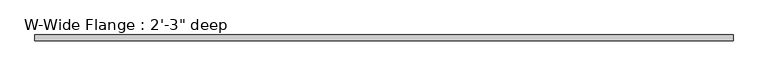
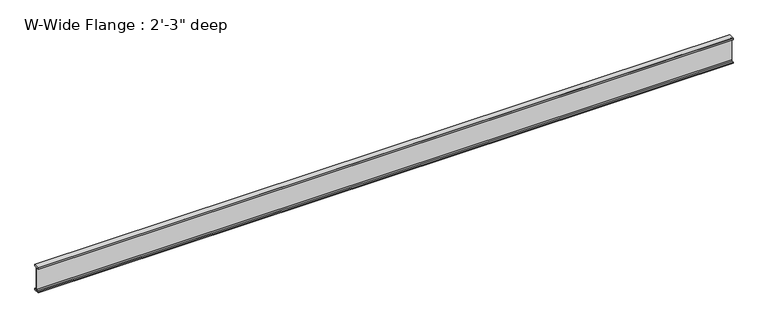
"""IFC4 building model written with IfcOpenShell, lengths in millimetres: beam geometry."""

import ifcopenshell
import ifcopenshell.guid

model = None  # the IFC model being written
_history = None  # IfcOwnerHistory: only IFC2X3 demands one
_inside = {}  # id of a spatial element -> (the spatial element, [elements in it])
_under = {}  # id of a project, library or spatial element -> (it, [spatial elements below it])
_declared = {}  # id of a project -> (the project, [libraries it declares])
_typed = {}  # id of a type object -> (the type object, [elements of that type])
_made_of = {}  # id of a material, layer set ... -> (it, [elements and type objects made of it])


def new_model(schema):
    """Start an empty IFC model of exactly this schema.

    Asked for "IFC4X3", IfcOpenShell would pick the latest addendum, in which some entities
    have other attributes; the version numbers below select the first issue.
    IFC2X3 requires an IfcOwnerHistory on every rooted entity: one is made here for all.
    """
    global model, _history
    if schema == "IFC4X3":
        model = ifcopenshell.file(schema_version=(4, 3, 0, 0))
    else:
        model = ifcopenshell.file(schema=schema)
    _inside.clear()
    _under.clear()
    _declared.clear()
    _typed.clear()
    _made_of.clear()
    _history = None
    if model.schema == "IFC2X3":
        org = make("IfcOrganization", Name="unknown")
        user = make(
            "IfcPersonAndOrganization",
            ThePerson=make("IfcPerson", FamilyName="unknown"),
            TheOrganization=org,
        )
        app = make(
            "IfcApplication",
            ApplicationDeveloper=org,
            Version="unknown",
            ApplicationFullName="unknown",
            ApplicationIdentifier="unknown",
        )
        _history = make(
            "IfcOwnerHistory",
            OwningUser=user,
            OwningApplication=app,
            ChangeAction="ADDED",
            CreationDate=0,
        )
    return model


def make(cls, **values):
    """One entity of the class cls with the attributes given. An attribute that is None is left unset."""
    return model.create_entity(
        cls, **{name: value for name, value in values.items() if value is not None}
    )


def rooted(cls, **values):
    """An entity with a GlobalId (a new one), such as an element, a storey or a relation."""
    return make(cls, GlobalId=ifcopenshell.guid.new(), OwnerHistory=_history, **values)


def si_unit(unit_type, name, prefix=None):
    """IfcSIUnit, for example si_unit("LENGTHUNIT", "METRE", prefix="MILLI")."""
    return make("IfcSIUnit", UnitType=unit_type, Prefix=prefix, Name=name)


def assignment(units):
    """IfcUnitAssignment: the units of a project."""
    return None if units is None else make("IfcUnitAssignment", Units=units)


def point(xyz):
    """IfcCartesianPoint."""
    return None if xyz is None else make("IfcCartesianPoint", Coordinates=xyz)


def direction(xyz):
    """IfcDirection."""
    return None if xyz is None else make("IfcDirection", DirectionRatios=xyz)


def frame(location, z_axis=None, x_axis=None):
    """IfcAxis2Placement3D, a coordinate frame: its origin and axes. An axis left out is left unset."""
    return make(
        "IfcAxis2Placement3D",
        Location=point(location),
        Axis=direction(z_axis),
        RefDirection=direction(x_axis),
    )


def frame_2d(location, x_axis=None):
    """IfcAxis2Placement2D, a coordinate frame in the plane: its origin and x axis."""
    return make(
        "IfcAxis2Placement2D", Location=point(location), RefDirection=direction(x_axis)
    )


def origin():
    """The frame at (0, 0, 0) with its axes left unset."""
    return frame((0.0, 0.0, 0.0))


def place(relative_to, where):
    """IfcLocalPlacement: puts the frame where relative to a parent placement (None: the world)."""
    return make(
        "IfcLocalPlacement", PlacementRelTo=relative_to, RelativePlacement=where
    )


def context(
    kind, dimensions, precision=None, world=None, true_north=None, identifier=None
):
    """IfcGeometricRepresentationContext, for example the 3D "Model" context."""
    return make(
        "IfcGeometricRepresentationContext",
        ContextIdentifier=identifier,
        ContextType=kind,
        CoordinateSpaceDimension=dimensions,
        Precision=precision,
        WorldCoordinateSystem=world,
        TrueNorth=true_north,
    )


def project(units=None, contexts=None):
    """IfcProject with its units and contexts."""
    return rooted(
        "IfcProject",
        Name="project",
        RepresentationContexts=contexts,
        UnitsInContext=assignment(units),
    )


def spatial(cls, under=None, at=None, **own):
    """A site, building, storey or space (cls), placed at a placement, below another one or the project."""
    s = rooted(cls, ObjectPlacement=at, **own)
    if under is not None:
        _under.setdefault(under.id(), (under, []))[1].append(s)
    return s


def polyline(points):
    """IfcPolyline through the points."""
    return make("IfcPolyline", Points=[point(p) for p in points])


def circle_curve(where, radius):
    """IfcCircle in the frame where."""
    return make("IfcCircle", Position=where, Radius=radius)


def trimmed(basis, trim1, trim2, sense, master):
    """IfcTrimmedCurve: the piece of a basis curve between two trims."""
    return make(
        "IfcTrimmedCurve",
        BasisCurve=basis,
        Trim1=trim1,
        Trim2=trim2,
        SenseAgreement=sense,
        MasterRepresentation=master,
    )


def segment(curve, same_sense, transition):
    """IfcCompositeCurveSegment."""
    return make(
        "IfcCompositeCurveSegment",
        Transition=transition,
        SameSense=same_sense,
        ParentCurve=curve,
    )


def composite_curve(segments, self_intersect=None):
    """IfcCompositeCurve: segments joined end to end."""
    return make("IfcCompositeCurve", Segments=segments, SelfIntersect=self_intersect)


def outline(outer, holes=None, kind="AREA"):
    """IfcArbitraryClosedProfileDef: a profile drawn as a closed curve; with holes, ...WithVoids."""
    if holes is None:
        return make("IfcArbitraryClosedProfileDef", ProfileType=kind, OuterCurve=outer)
    return make(
        "IfcArbitraryProfileDefWithVoids",
        ProfileType=kind,
        OuterCurve=outer,
        InnerCurves=holes,
    )


def extrude(swept, where, along, depth):
    """IfcExtrudedAreaSolid: the profile swept, set in the frame where, extruded along a direction by depth."""
    return make(
        "IfcExtrudedAreaSolid",
        SweptArea=swept,
        Position=where,
        ExtrudedDirection=direction(along),
        Depth=depth,
    )


def shape(context_of_items, identifier, shape_type, items):
    """IfcShapeRepresentation: the items that make up one representation, for example the "Body"."""
    return make(
        "IfcShapeRepresentation",
        ContextOfItems=context_of_items,
        RepresentationIdentifier=identifier,
        RepresentationType=shape_type,
        Items=items,
    )


def source(mapping_origin, context_of_items, identifier, shape_type, items):
    """IfcRepresentationMap: a shape defined once, which mapped items show again and again."""
    return make(
        "IfcRepresentationMap",
        MappingOrigin=mapping_origin,
        MappedRepresentation=shape(context_of_items, identifier, shape_type, items),
    )


def transform(
    local_origin,
    x_axis=None,
    y_axis=None,
    z_axis=None,
    scale=None,
    scale2=None,
    scale3=None,
    uniform=True,
):
    """IfcCartesianTransformationOperator3D, or its non-uniform kind. x_axis, y_axis, z_axis: its Axis1, 2, 3."""
    if uniform:
        return make(
            "IfcCartesianTransformationOperator3D",
            Axis1=direction(x_axis),
            Axis2=direction(y_axis),
            LocalOrigin=point(local_origin),
            Scale=scale,
            Axis3=direction(z_axis),
        )
    return make(
        "IfcCartesianTransformationOperator3DnonUniform",
        Axis1=direction(x_axis),
        Axis2=direction(y_axis),
        LocalOrigin=point(local_origin),
        Scale=scale,
        Axis3=direction(z_axis),
        Scale2=scale2,
        Scale3=scale3,
    )


def mapped(mapping_source, mapping_target):
    """IfcMappedItem: shows the shape of a source again, moved by a transform."""
    return make(
        "IfcMappedItem", MappingSource=mapping_source, MappingTarget=mapping_target
    )


def made_of(thing, what):
    """Note that an element or type object is made of a material, layer set ...; save() writes the relation."""
    if what is not None:
        _made_of.setdefault(what.id(), (what, []))[1].append(thing)
    return thing


def element(
    cls,
    number,
    at=None,
    inside=None,
    cuts=None,
    type_object=None,
    material=None,
    context=None,
    identifier="Body",
    shape_type=None,
    held_by="IfcProductDefinitionShape",
    body=None,
    shapes=None,
    **own,
):
    """One element of the class cls, such as IfcWall. Its Tag is "e" and its number.

    at: its placement. inside: the storey or other place that contains it. cuts: it is an
    opening in that element (IfcRelVoidsElement). A single representation is given by context,
    identifier, shape_type and body (its items); several are given by shapes. held_by: the class
    of the entity that holds the representations. save() writes the other relations.
    """
    e = rooted(cls, Tag="e%d" % number, ObjectPlacement=at, **own)
    if body is not None:
        shapes = [shape(context, identifier, shape_type, body)]
    if shapes is not None:
        e.Representation = make(held_by, Representations=shapes)
    if inside is not None:
        _inside.setdefault(inside.id(), (inside, []))[1].append(e)
    if cuts is not None:
        rooted(
            "IfcRelVoidsElement", RelatingBuildingElement=cuts, RelatedOpeningElement=e
        )
    if type_object is not None:
        _typed.setdefault(type_object.id(), (type_object, []))[1].append(e)
    return made_of(e, material)


def aggregate(whole, parts):
    """IfcRelAggregates: a whole, such as a stair, and the parts it consists of."""
    return rooted("IfcRelAggregates", RelatingObject=whole, RelatedObjects=parts)


def save(model, path):
    """Write the relations noted so far, then the file.

    IfcRelAggregates (storeys below a building ...), IfcRelContainedInSpatialStructure (elements
    in a storey), IfcRelDefinesByType, IfcRelAssociatesMaterial and IfcRelDeclares: one each for
    every whole, place, type object, material and project.
    """
    for whole, parts in _under.values():
        aggregate(whole, parts)
    for where, things in _inside.values():
        rooted(
            "IfcRelContainedInSpatialStructure",
            RelatedElements=things,
            RelatingStructure=where,
        )
    for kind, things in _typed.values():
        rooted("IfcRelDefinesByType", RelatedObjects=things, RelatingType=kind)
    for what, things in _made_of.values():
        rooted("IfcRelAssociatesMaterial", RelatedObjects=things, RelatingMaterial=what)
    for by, libraries in _declared.values():
        rooted("IfcRelDeclares", RelatingContext=by, RelatedDefinitions=libraries)
    model.write(path)


def beam_74707e8d(model_context):
    return source(origin(), model_context, "Body", "SweptSolid", [
        extrude(outline(composite_curve([segment(polyline([(76.2, -308.356), (76.2, -342.9), (-76.2, -342.9), (-76.2, -308.356), (-32.131, -308.356)]), True, "CONTINUOUS"), segment(trimmed(circle_curve(frame_2d((-32.131, -285.75)), 22.606), [point((-32.131, -308.356))], [point((-9.525, -285.75))], True, "CARTESIAN"), True, "CONTINUOUS"), segment(polyline([(-9.525, -285.75), (-9.525, 285.75)]), True, "CONTINUOUS"), segment(trimmed(circle_curve(frame_2d((-32.131, 285.75)), 22.606), [point((-9.525, 285.75))], [point((-32.131, 308.356))], True, "CARTESIAN"), True, "CONTINUOUS"), segment(polyline([(-32.131, 308.356), (-76.2, 308.356), (-76.2, 342.9), (76.2, 342.9), (76.2, 308.356), (32.131, 308.356)]), True, "CONTINUOUS"), segment(trimmed(circle_curve(frame_2d((32.131, 285.75)), 22.606), [point((32.131, 308.356))], [point((9.525, 285.75))], True, "CARTESIAN"), True, "CONTINUOUS"), segment(polyline([(9.525, 285.75), (9.525, -285.75)]), True, "CONTINUOUS"), segment(trimmed(circle_curve(frame_2d((32.131, -285.75)), 22.606), [point((9.525, -285.75))], [point((32.131, -308.356))], True, "CARTESIAN"), True, "CONTINUOUS"), segment(polyline([(32.131, -308.356), (76.2, -308.356)]), True, "CONTINUOUS")], self_intersect=False)), frame((-8971.3142226, 0.0, 0.0), z_axis=(1.0, 0.0, 0.0), x_axis=(0.0, 1.0, 0.0)), (0.0, 0.0, 1.0), 17940.5898041),
    ])


if __name__ == "__main__":
    model = new_model("IFC4")
    model_context = context("Model", 3, world=origin())
    ifc_project = project(units=[si_unit("LENGTHUNIT", "METRE", prefix="MILLI")], contexts=[model_context])
    site = spatial("IfcSite", under=ifc_project)
    building = spatial("IfcBuilding", under=site)
    placement = place(None, origin())
    beam_shape = beam_74707e8d(model_context)
    element("IfcBeam", 1, ObjectType="W-Wide Flange : 2'-3\" deep", at=placement, inside=building, context=model_context, shape_type="MappedRepresentation", body=[
        mapped(beam_shape, transform((0.0, 0.0, 0.0), x_axis=(1.0, 0.0, 0.0), y_axis=(0.0, 1.0, 0.0), z_axis=(0.0, 0.0, 1.0))),
    ])
    save(model, "model.ifc")

# Revit data of these elements
# Type "W-Wide Flange : 2'-3\" deep"
#   Assembly Code = "B10"
#   W = 166
#   Length [instance default] = 5' - 0"
#   bf = 0' - 6"
#   d = 2' - 3"
#   k = 0' - 2 1/4"
#   k2 = 0' - 0.89"
#   tf = 0' - 1.36"
#   tw = 0' - 0 3/4"
#   A = 0.338889 SF
#   Structural Material [instance default] = Steel ASTM A992
# Element 1 (IfcBeam, "W-Wide Flange : 2'-3\" deep")
#   Structural Material = STRUCTURAL STEEL - SEE STRUCT. DWGS
#   Materials on its faces: "STRUCTURAL STEEL - SEE STRUCT. DWGS"
# Materials
#   "Steel ASTM A992": class "Metal", colour RGB 199 199 199, transparency 0, Description = "Structural steel 50ksi", Cost = 0
#   "STRUCTURAL STEEL - SEE STRUCT. DWGS": class "Metal", colour RGB 137 146 153, transparency 0, Description = "Steel, mill finish", Cost = 0
